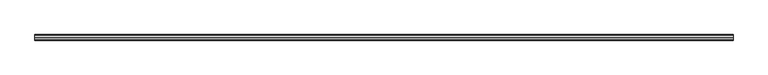
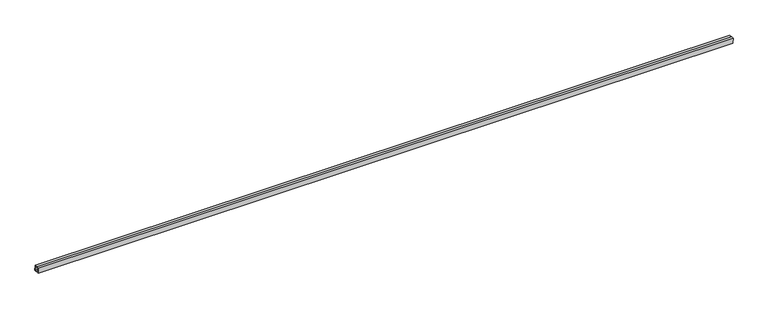
"""IFC4 building model written with IfcOpenShell, lengths in millimetres: proxy geometry, Inner panel:Inner panel:1:Inner panel:1 : Inner panel:Inner panel:300324:2:Inner panel:1:Inner panel:1 : Inner panel:Inner panel:300324:2 : Inner panel:Inner panel:1:Inner panel:1 : Inner panel:Inner panel:300324:300043:28 : Inner panel:Inner panel:1:Inner panel:1 : Inner panel:Inner panel:300324:2:Inner panel:1:Inner panel:1 : Inner panel:Inner panel:300324:2 : Inner panel:Inner panel:1:Inner panel:1 : Inner panel:Inner panel:300324:300043:308120."""

from ifc_helpers import new_model, si_unit, frame, origin, place, context, project, spatial, polyline, outline, extrude, source, transform, mapped, element, save


def generic_models_e1ab8ac2(model_context):
    return source(origin(), model_context, "Body", "SweptSolid", [
        extrude(outline(polyline([(-565838.6723382, 8901.5279981), (-565820.431915, 8902.2880157), (-565818.8457913, 8864.2210456), (-565856.9127614, 8862.6349219), (-565858.4988851, 8900.701892), (-565840.2584619, 8901.4619096), (-565840.1593292, 8899.082724), (-565856.0205667, 8898.4218391), (-565854.6327085, 8865.1132403), (-565821.3241096, 8866.5010985), (-565822.7119679, 8899.8096974), (-565838.5732055, 8899.1488125), (-565838.6723382, 8901.5279981)])), frame((588245.3367242, 0.0, 0.0), z_axis=(1.0, 0.0, 0.0), x_axis=(0.0, 1.0, 0.0)), (0.0, 0.0, 1.0), 4876.8),
    ])


if __name__ == "__main__":
    model = new_model("IFC4")
    model_context = context("Model", 3, world=origin())
    ifc_project = project(units=[si_unit("LENGTHUNIT", "METRE", prefix="MILLI")], contexts=[model_context])
    site = spatial("IfcSite", under=ifc_project)
    building = spatial("IfcBuilding", under=site)
    placement = place(None, origin())
    generic_models_shape = generic_models_e1ab8ac2(model_context)
    element("IfcBuildingElementProxy", 1, Name="Inner panel:Inner panel:1:Inner panel:1 : Inner panel:Inner panel:300324:2:Inner panel:1:Inner panel:1 : Inner panel:Inner panel:300324:2 : Inner panel:Inner panel:1:Inner panel:1 : Inner panel:Inner panel:300324:300043:28 : Inner panel:Inner panel:1:Inner panel:1 : Inner panel:Inner panel:300324:2:Inner panel:1:Inner panel:1 : Inner panel:Inner panel:300324:2 : Inner panel:Inner panel:1:Inner panel:1 : Inner panel:Inner panel:300324:300043:308120", ObjectType="Inner panel:Inner panel:1:Inner panel:1 : Inner panel:Inner panel:300324:2:Inner panel:1:Inner panel:1 : Inner panel:Inner panel:300324:2 : Inner panel:Inner panel:1:Inner panel:1 : Inner panel:Inner panel:300324:300043:28 : Inner panel:Inner panel:1:Inner panel:1 : Inner panel:Inner panel:300324:2:Inner panel:1:Inner panel:1 : Inner panel:Inner panel:300324:2 : Inner panel:Inner panel:1:Inner panel:1 : Inner panel:Inner panel:300324:300043:308120", at=placement, inside=building, context=model_context, shape_type="MappedRepresentation", body=[
        mapped(generic_models_shape, transform((0.0, 0.0, 0.0), x_axis=(1.0, 0.0, 0.0), y_axis=(0.0, 1.0, 0.0), z_axis=(0.0, 0.0, 1.0))),
    ])
    save(model, "model.ifc")

# Revit data of these elements
# Type "Inner panel:Inner panel:1:Inner panel:1 : Inner panel:Inner panel:300324:2:Inner panel:1:Inner panel:1 : Inner panel:Inner panel:300324:2 : Inner panel:Inner panel:1:Inner panel:1 : Inner panel:Inner panel:300324:300043:28 : Inner panel:Inner panel:1:Inner panel:1 : Inner panel:Inner panel:300324:2:Inner panel:1:Inner panel:1 : Inner panel:Inner panel:300324:2 : Inner panel:Inner panel:1:Inner panel:1 : Inner panel:Inner panel:300324:300043:308120"
#   NameOverride = "Inner panel:Inner panel:1:Inner panel:1 : Inner panel:Inner panel:300324:2:Inner panel:1:Inner panel:1 : Inner panel:Inner panel:300324:2 : Inner panel:Inner panel:1:Inner panel:1 : Inner panel:Inner panel:300324:300043:308120"
#   ObjectTypeOverride = "Inner panel:1:Inner panel:1 : Inner panel:Inner panel:300324:2 : Inner panel:Inner panel:1:Inner panel:1 : Inner panel:Inner panel:300324:300043"
#   Reference = "Inner panel"
#   Tag = "308120"
# Element 1 (IfcBuildingElementProxy, "Inner panel:Inner panel:1:Inner panel:1 : Inner panel:Inner panel:300324:2:Inner panel:1:Inner panel:1 : Inner panel:Inner panel:300324:2 : Inner panel:Inner panel:1:Inner panel:1 : Inner panel:Inner panel:300324:300043:28 : Inner panel:Inner panel:1:Inner panel:1 : Inner panel:Inner panel:300324:2:Inner panel:1:Inner panel:1 : Inner panel:Inner panel:300324:2 : Inner panel:Inner panel:1:Inner panel:1 : Inner panel:Inner panel:300324:300043:308120")
#   Materials on its faces: "1 1/2\" X 1 1/2\" SPLIT-SEAM SQUARE TUBING (~24\" CANTILEVER FROM C.L. OF GLULAM)"
# Materials
#   "1 1/2\" X 1 1/2\" SPLIT-SEAM SQUARE TUBING (~24\" CANTILEVER FROM C.L. OF GLULAM)": class "Unassigned", colour RGB 202 201 200, transparency 0, Cost = 0
